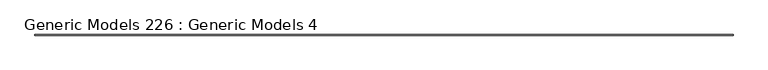
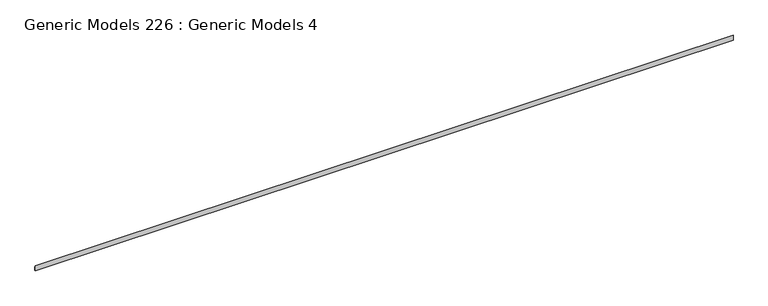
"""IFC4 building model written with IfcOpenShell, lengths in millimetres: proxy geometry, Generic Models 226 : Generic Models 4."""

from ifc_helpers import new_model, si_unit, frame, origin, place, context, project, spatial, polyline, outline, extrude, source, transform, mapped, element, save


def generic_models_226_generic_models_4_14ee75c6(model_context):
    return source(origin(), model_context, "Body", "SweptSolid", [
        extrude(outline(polyline([(-29346.0685041, 127006.935011), (-29363.8485041, 127001.220011), (-29363.8485041, 127143.9556439), (-29346.0685041, 127109.3314334), (-29346.0685041, 127006.935011)])), frame((-20795.7733045, 0.0, 0.0), z_axis=(1.0, 0.0, 0.0), x_axis=(0.0, 1.0, 0.0)), (0.0, 0.0, 1.0), 18643.6),
    ])


if __name__ == "__main__":
    model = new_model("IFC4")
    model_context = context("Model", 3, world=origin())
    ifc_project = project(units=[si_unit("LENGTHUNIT", "METRE", prefix="MILLI")], contexts=[model_context])
    site = spatial("IfcSite", under=ifc_project)
    building = spatial("IfcBuilding", under=site)
    placement = place(None, origin())
    generic_models_226_generic_models_4_shape = generic_models_226_generic_models_4_14ee75c6(model_context)
    element("IfcBuildingElementProxy", 1, Name="Generic Models 226 : Generic Models 4", ObjectType="Generic Models 226 : Generic Models 4", at=placement, inside=building, context=model_context, shape_type="MappedRepresentation", body=[
        mapped(generic_models_226_generic_models_4_shape, transform((0.0, 0.0, 0.0), x_axis=(1.0, 0.0, 0.0), y_axis=(0.0, 1.0, 0.0), z_axis=(0.0, 0.0, 1.0))),
    ])
    save(model, "model.ifc")

# Revit data of these elements
# Element 1 (IfcBuildingElementProxy, "Generic Models 226 : Generic Models 4")
#   Materials on its faces: "_7/8\" SMOOTH TROWEL EXTERIOR STUCCO (COLOR PER OWNER)"
# Materials
#   "_7/8\" SMOOTH TROWEL EXTERIOR STUCCO (COLOR PER OWNER)": class "Generic", colour RGB 233 233 233, transparency 0, Cost = 0
